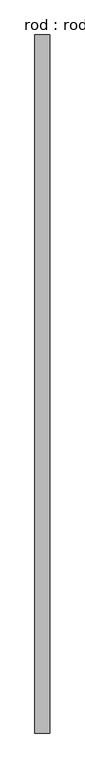
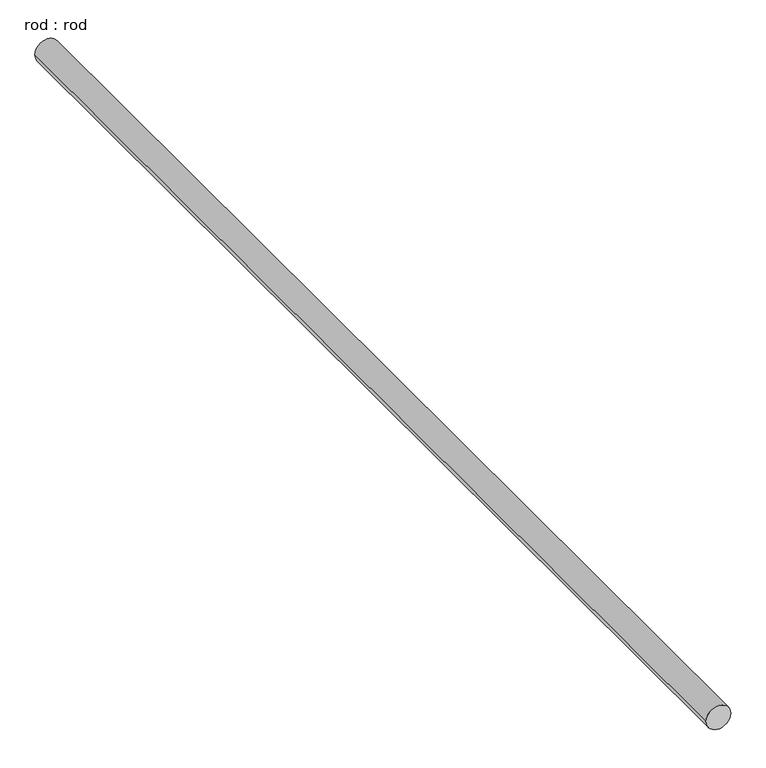
"""IFC4 building model written with IfcOpenShell, lengths in millimetres: proxy geometry, rod : rod."""

from ifc_helpers import new_model, si_unit, point, frame, frame_2d, origin, place, context, project, spatial, circle_curve, trimmed, segment, composite_curve, outline, extrude, source, transform, mapped, element, save


def rod_rod_5b2441ec(model_context):
    return source(origin(), model_context, "Body", "SweptSolid", [
        extrude(outline(composite_curve([segment(trimmed(circle_curve(frame_2d((0.0108462, 0.0)), 200.0), [point((0.0108462, 200.0))], [point((0.0108462, -200.0))], False, "CARTESIAN"), True, "CONTINUOUS"), segment(trimmed(circle_curve(frame_2d((0.0108462, 0.0)), 200.0), [point((0.0108462, -200.0))], [point((0.0108462, 200.0))], False, "CARTESIAN"), True, "CONTINUOUS")], self_intersect=False)), frame((0.0, -5335.8428132, 0.0), z_axis=(0.0, 1.0, 0.0), x_axis=(0.0, 0.0, 1.0)), (0.0, 0.0, 1.0), 18857.1428571),
    ])


if __name__ == "__main__":
    model = new_model("IFC4")
    model_context = context("Model", 3, world=origin())
    ifc_project = project(units=[si_unit("LENGTHUNIT", "METRE", prefix="MILLI")], contexts=[model_context])
    site = spatial("IfcSite", under=ifc_project)
    building = spatial("IfcBuilding", under=site)
    placement = place(None, origin())
    rod_rod_shape = rod_rod_5b2441ec(model_context)
    element("IfcBuildingElementProxy", 1, Name="rod : rod", ObjectType="rod : rod", at=placement, inside=building, context=model_context, shape_type="MappedRepresentation", body=[
        mapped(rod_rod_shape, transform((0.0, 0.0, 0.0), x_axis=(1.0, 0.0, 0.0), y_axis=(0.0, 1.0, 0.0), z_axis=(0.0, 0.0, 1.0))),
    ])
    save(model, "model.ifc")

# Revit data of these elements
# Type "rod : rod"
#   Default Elevation = 0
